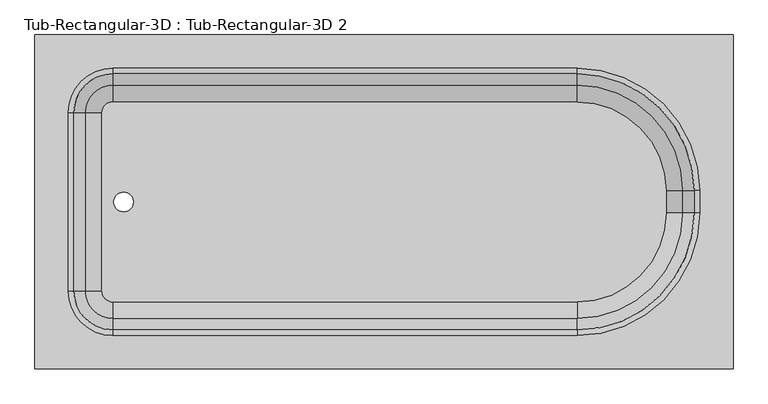
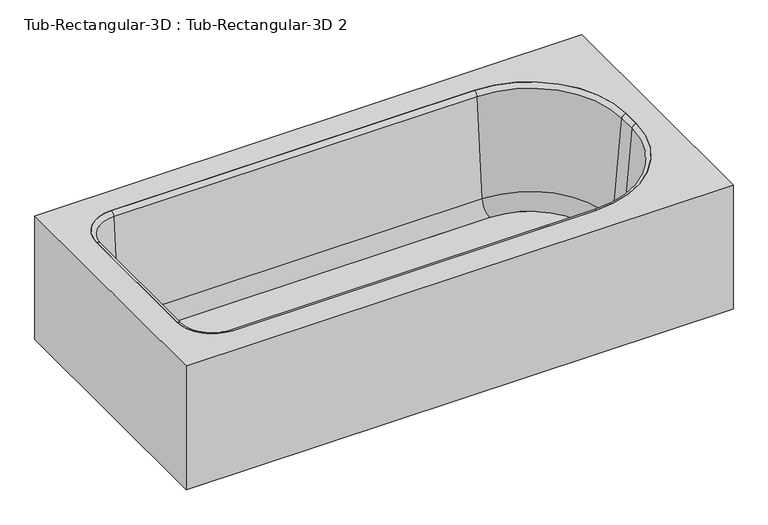
"""IFC4 building model written with IfcOpenShell, lengths in millimetres: flow terminal geometry, Tub-Rectangular-3D : Tub-Rectangular-3D 2."""

import ifcopenshell
import ifcopenshell.guid

model = None  # the IFC model being written
_history = None  # IfcOwnerHistory: only IFC2X3 demands one
_inside = {}  # id of a spatial element -> (the spatial element, [elements in it])
_under = {}  # id of a project, library or spatial element -> (it, [spatial elements below it])
_declared = {}  # id of a project -> (the project, [libraries it declares])
_typed = {}  # id of a type object -> (the type object, [elements of that type])
_made_of = {}  # id of a material, layer set ... -> (it, [elements and type objects made of it])


def new_model(schema):
    """Start an empty IFC model of exactly this schema.

    Asked for "IFC4X3", IfcOpenShell would pick the latest addendum, in which some entities
    have other attributes; the version numbers below select the first issue.
    IFC2X3 requires an IfcOwnerHistory on every rooted entity: one is made here for all.
    """
    global model, _history
    if schema == "IFC4X3":
        model = ifcopenshell.file(schema_version=(4, 3, 0, 0))
    else:
        model = ifcopenshell.file(schema=schema)
    _inside.clear()
    _under.clear()
    _declared.clear()
    _typed.clear()
    _made_of.clear()
    _history = None
    if model.schema == "IFC2X3":
        org = make("IfcOrganization", Name="unknown")
        user = make(
            "IfcPersonAndOrganization",
            ThePerson=make("IfcPerson", FamilyName="unknown"),
            TheOrganization=org,
        )
        app = make(
            "IfcApplication",
            ApplicationDeveloper=org,
            Version="unknown",
            ApplicationFullName="unknown",
            ApplicationIdentifier="unknown",
        )
        _history = make(
            "IfcOwnerHistory",
            OwningUser=user,
            OwningApplication=app,
            ChangeAction="ADDED",
            CreationDate=0,
        )
    return model


def make(cls, **values):
    """One entity of the class cls with the attributes given. An attribute that is None is left unset."""
    return model.create_entity(
        cls, **{name: value for name, value in values.items() if value is not None}
    )


def rooted(cls, **values):
    """An entity with a GlobalId (a new one), such as an element, a storey or a relation."""
    return make(cls, GlobalId=ifcopenshell.guid.new(), OwnerHistory=_history, **values)


def si_unit(unit_type, name, prefix=None):
    """IfcSIUnit, for example si_unit("LENGTHUNIT", "METRE", prefix="MILLI")."""
    return make("IfcSIUnit", UnitType=unit_type, Prefix=prefix, Name=name)


def assignment(units):
    """IfcUnitAssignment: the units of a project."""
    return None if units is None else make("IfcUnitAssignment", Units=units)


def point(xyz):
    """IfcCartesianPoint."""
    return None if xyz is None else make("IfcCartesianPoint", Coordinates=xyz)


def direction(xyz):
    """IfcDirection."""
    return None if xyz is None else make("IfcDirection", DirectionRatios=xyz)


def frame(location, z_axis=None, x_axis=None):
    """IfcAxis2Placement3D, a coordinate frame: its origin and axes. An axis left out is left unset."""
    return make(
        "IfcAxis2Placement3D",
        Location=point(location),
        Axis=direction(z_axis),
        RefDirection=direction(x_axis),
    )


def frame_2d(location, x_axis=None):
    """IfcAxis2Placement2D, a coordinate frame in the plane: its origin and x axis."""
    return make(
        "IfcAxis2Placement2D", Location=point(location), RefDirection=direction(x_axis)
    )


def origin():
    """The frame at (0, 0, 0) with its axes left unset."""
    return frame((0.0, 0.0, 0.0))


def place(relative_to, where):
    """IfcLocalPlacement: puts the frame where relative to a parent placement (None: the world)."""
    return make(
        "IfcLocalPlacement", PlacementRelTo=relative_to, RelativePlacement=where
    )


def context(
    kind, dimensions, precision=None, world=None, true_north=None, identifier=None
):
    """IfcGeometricRepresentationContext, for example the 3D "Model" context."""
    return make(
        "IfcGeometricRepresentationContext",
        ContextIdentifier=identifier,
        ContextType=kind,
        CoordinateSpaceDimension=dimensions,
        Precision=precision,
        WorldCoordinateSystem=world,
        TrueNorth=true_north,
    )


def project(units=None, contexts=None):
    """IfcProject with its units and contexts."""
    return rooted(
        "IfcProject",
        Name="project",
        RepresentationContexts=contexts,
        UnitsInContext=assignment(units),
    )


def spatial(cls, under=None, at=None, **own):
    """A site, building, storey or space (cls), placed at a placement, below another one or the project."""
    s = rooted(cls, ObjectPlacement=at, **own)
    if under is not None:
        _under.setdefault(under.id(), (under, []))[1].append(s)
    return s


def polyline(points):
    """IfcPolyline through the points."""
    return make("IfcPolyline", Points=[point(p) for p in points])


def circle_curve(where, radius):
    """IfcCircle in the frame where."""
    return make("IfcCircle", Position=where, Radius=radius)


def ellipse_curve(where, semi_axis1, semi_axis2):
    """IfcEllipse in the frame where."""
    return make(
        "IfcEllipse", Position=where, SemiAxis1=semi_axis1, SemiAxis2=semi_axis2
    )


def trimmed(basis, trim1, trim2, sense, master):
    """IfcTrimmedCurve: the piece of a basis curve between two trims."""
    return make(
        "IfcTrimmedCurve",
        BasisCurve=basis,
        Trim1=trim1,
        Trim2=trim2,
        SenseAgreement=sense,
        MasterRepresentation=master,
    )


def segment(curve, same_sense, transition):
    """IfcCompositeCurveSegment."""
    return make(
        "IfcCompositeCurveSegment",
        Transition=transition,
        SameSense=same_sense,
        ParentCurve=curve,
    )


def composite_curve(segments, self_intersect=None):
    """IfcCompositeCurve: segments joined end to end."""
    return make("IfcCompositeCurve", Segments=segments, SelfIntersect=self_intersect)


def outline(outer, holes=None, kind="AREA"):
    """IfcArbitraryClosedProfileDef: a profile drawn as a closed curve; with holes, ...WithVoids."""
    if holes is None:
        return make("IfcArbitraryClosedProfileDef", ProfileType=kind, OuterCurve=outer)
    return make(
        "IfcArbitraryProfileDefWithVoids",
        ProfileType=kind,
        OuterCurve=outer,
        InnerCurves=holes,
    )


def extrude(swept, where, along, depth):
    """IfcExtrudedAreaSolid: the profile swept, set in the frame where, extruded along a direction by depth."""
    return make(
        "IfcExtrudedAreaSolid",
        SweptArea=swept,
        Position=where,
        ExtrudedDirection=direction(along),
        Depth=depth,
    )


def shape(context_of_items, identifier, shape_type, items):
    """IfcShapeRepresentation: the items that make up one representation, for example the "Body"."""
    return make(
        "IfcShapeRepresentation",
        ContextOfItems=context_of_items,
        RepresentationIdentifier=identifier,
        RepresentationType=shape_type,
        Items=items,
    )


def source(mapping_origin, context_of_items, identifier, shape_type, items):
    """IfcRepresentationMap: a shape defined once, which mapped items show again and again."""
    return make(
        "IfcRepresentationMap",
        MappingOrigin=mapping_origin,
        MappedRepresentation=shape(context_of_items, identifier, shape_type, items),
    )


def transform(
    local_origin,
    x_axis=None,
    y_axis=None,
    z_axis=None,
    scale=None,
    scale2=None,
    scale3=None,
    uniform=True,
):
    """IfcCartesianTransformationOperator3D, or its non-uniform kind. x_axis, y_axis, z_axis: its Axis1, 2, 3."""
    if uniform:
        return make(
            "IfcCartesianTransformationOperator3D",
            Axis1=direction(x_axis),
            Axis2=direction(y_axis),
            LocalOrigin=point(local_origin),
            Scale=scale,
            Axis3=direction(z_axis),
        )
    return make(
        "IfcCartesianTransformationOperator3DnonUniform",
        Axis1=direction(x_axis),
        Axis2=direction(y_axis),
        LocalOrigin=point(local_origin),
        Scale=scale,
        Axis3=direction(z_axis),
        Scale2=scale2,
        Scale3=scale3,
    )


def mapped(mapping_source, mapping_target):
    """IfcMappedItem: shows the shape of a source again, moved by a transform."""
    return make(
        "IfcMappedItem", MappingSource=mapping_source, MappingTarget=mapping_target
    )


def made_of(thing, what):
    """Note that an element or type object is made of a material, layer set ...; save() writes the relation."""
    if what is not None:
        _made_of.setdefault(what.id(), (what, []))[1].append(thing)
    return thing


def element(
    cls,
    number,
    at=None,
    inside=None,
    cuts=None,
    type_object=None,
    material=None,
    context=None,
    identifier="Body",
    shape_type=None,
    held_by="IfcProductDefinitionShape",
    body=None,
    shapes=None,
    **own,
):
    """One element of the class cls, such as IfcWall. Its Tag is "e" and its number.

    at: its placement. inside: the storey or other place that contains it. cuts: it is an
    opening in that element (IfcRelVoidsElement). A single representation is given by context,
    identifier, shape_type and body (its items); several are given by shapes. held_by: the class
    of the entity that holds the representations. save() writes the other relations.
    """
    e = rooted(cls, Tag="e%d" % number, ObjectPlacement=at, **own)
    if body is not None:
        shapes = [shape(context, identifier, shape_type, body)]
    if shapes is not None:
        e.Representation = make(held_by, Representations=shapes)
    if inside is not None:
        _inside.setdefault(inside.id(), (inside, []))[1].append(e)
    if cuts is not None:
        rooted(
            "IfcRelVoidsElement", RelatingBuildingElement=cuts, RelatedOpeningElement=e
        )
    if type_object is not None:
        _typed.setdefault(type_object.id(), (type_object, []))[1].append(e)
    return made_of(e, material)


def aggregate(whole, parts):
    """IfcRelAggregates: a whole, such as a stair, and the parts it consists of."""
    return rooted("IfcRelAggregates", RelatingObject=whole, RelatedObjects=parts)


def save(model, path):
    """Write the relations noted so far, then the file.

    IfcRelAggregates (storeys below a building ...), IfcRelContainedInSpatialStructure (elements
    in a storey), IfcRelDefinesByType, IfcRelAssociatesMaterial and IfcRelDeclares: one each for
    every whole, place, type object, material and project.
    """
    for whole, parts in _under.values():
        aggregate(whole, parts)
    for where, things in _inside.values():
        rooted(
            "IfcRelContainedInSpatialStructure",
            RelatedElements=things,
            RelatingStructure=where,
        )
    for kind, things in _typed.values():
        rooted("IfcRelDefinesByType", RelatedObjects=things, RelatingType=kind)
    for what, things in _made_of.values():
        rooted("IfcRelAssociatesMaterial", RelatedObjects=things, RelatingMaterial=what)
    for by, libraries in _declared.values():
        rooted("IfcRelDeclares", RelatingContext=by, RelatedDefinitions=libraries)
    model.write(path)


def plane_surface(at):
    """IfcPlane: the flat surface through the origin of the frame at, square to its z axis."""
    return make("IfcPlane", Position=at)


def cylinder_surface(at, radius):
    """IfcCylindricalSurface: all points at the distance radius from the z axis of the frame at."""
    return make("IfcCylindricalSurface", Position=at, Radius=radius)


def revolved_surface(curve, axis_point, axis_direction):
    """IfcSurfaceOfRevolution: the curve turned about the line through axis_point along axis_direction."""
    return make(
        "IfcSurfaceOfRevolution",
        SweptCurve=make("IfcArbitraryOpenProfileDef", ProfileType="CURVE", Curve=curve),
        AxisPosition=make("IfcAxis1Placement", Location=point(axis_point), Axis=direction(axis_direction)),
    )


def advanced_brep(points, edges, surfaces, faces):
    """IfcAdvancedBrep: a solid bounded by faces that lie on surfaces and meet in shared edges.

    An edge is (start, end): straight between two places in points (the first is 0);
    or (start, end, curve); or (start, end, curve, False) where it runs against its curve.
    A face is (place in surfaces, loops), or (place, loops, False) where it looks against
    its surface's normal. A loop lists edges by number (the first is 1), with a minus sign
    where the edge is run from its end to its start. The first loop is the outer one.
    """
    corners = [point(p) for p in points]
    vertices = [make("IfcVertexPoint", VertexGeometry=c) for c in corners]
    made = []
    for start, end, *more in edges:
        made.append(
            make(
                "IfcEdgeCurve",
                EdgeStart=vertices[start],
                EdgeEnd=vertices[end],
                EdgeGeometry=more[0] if more else make("IfcPolyline", Points=[corners[start], corners[end]]),
                SameSense=more[1] if len(more) > 1 else True,
            )
        )
    hull = []
    for where, loops, *sense in faces:
        bounds = []
        for j, loop in enumerate(loops):
            ring = [make("IfcOrientedEdge", EdgeElement=made[abs(k) - 1], Orientation=k > 0) for k in loop]
            bounds.append(
                make(
                    "IfcFaceOuterBound" if j == 0 else "IfcFaceBound",
                    Bound=make("IfcEdgeLoop", EdgeList=ring),
                    Orientation=True,
                )
            )
        hull.append(make("IfcAdvancedFace", Bounds=bounds, FaceSurface=surfaces[where], SameSense=sense[0] if sense else True))
    return make("IfcAdvancedBrep", Outer=make("IfcClosedShell", CfsFaces=hull))


def tub_rectangular_3d_tub_rectangular_3d_2_b18e5bc2(model_context):
    return source(origin(), model_context, "Body", "SolidModel", [
        advanced_brep(
        [(480.0720313, 830.2625, 381.0), (-1110.6029687, 830.2625, 381.0), (-1110.6029687, 68.2625, 381.0), (480.0720313, 68.2625, 381.0), (-932.8029687, 754.0625, 381.0), (124.4720313, 754.0625, 381.0), (403.8720313, 474.6625, 381.0), (403.8720313, 423.8625, 381.0), (124.4720313, 144.4625, 381.0), (-932.8029687, 144.4625, 381.0), (-1034.4029687, 246.0625, 381.0), (-1034.4029687, 652.4625, 381.0), (461.0220313, 811.2125, 361.95), (461.0220313, 87.3125, 361.95), (-1091.5529687, 87.3125, 361.95), (-1091.5529687, 811.2125, 361.95), (-932.8029687, 754.0625, 361.95), (-1034.4029687, 652.4625, 361.95), (-1034.4029687, 246.0625, 361.95), (-932.8029687, 144.4625, 361.95), (124.4720313, 144.4625, 361.95), (403.8720313, 423.8625, 361.95), (403.8720313, 474.6625, 361.95), (124.4720313, 754.0625, 361.95), (480.0720313, 830.2625, 0.0), (-1110.6029687, 830.2625, 0.0), (-1110.6029687, 68.2625, 0.0), (480.0720313, 68.2625, 0.0), (461.0220313, 811.2125, 0.0), (-1091.5529687, 811.2125, 0.0), (-1091.5529687, 87.3125, 0.0), (461.0220313, 87.3125, 0.0)],
        [
            (0, 1),
            (1, 2),
            (2, 3),
            (3, 0),
            (4, 5),
            (5, 6, circle_curve(frame((124.4720313, 474.6625, 381.0), z_axis=(0.0, 0.0, -1.0), x_axis=(0.0, 1.0, 0.0)), 279.4)),
            (6, 7),
            (7, 8, circle_curve(frame((124.4720313, 423.8625, 381.0), z_axis=(0.0, 0.0, -1.0), x_axis=(0.0, 1.0, 0.0)), 279.4)),
            (8, 9),
            (9, 10, circle_curve(frame((-932.8029687, 246.0625, 381.0), z_axis=(0.0, 0.0, -1.0), x_axis=(0.0, 1.0, 0.0)), 101.6)),
            (10, 11),
            (11, 4, circle_curve(frame((-932.8029687, 652.4625, 381.0), z_axis=(0.0, 0.0, -1.0), x_axis=(0.0, 1.0, 0.0)), 101.6)),
            (12, 13),
            (13, 14),
            (14, 15),
            (15, 12),
            (16, 17, circle_curve(frame((-932.8029687, 652.4625, 361.95), z_axis=(0.0, 0.0, 1.0), x_axis=(0.0, 1.0, 0.0)), 101.6)),
            (17, 18),
            (18, 19, circle_curve(frame((-932.8029687, 246.0625, 361.95), z_axis=(0.0, 0.0, 1.0), x_axis=(0.0, 1.0, 0.0)), 101.6)),
            (19, 20),
            (20, 21, circle_curve(frame((124.4720313, 423.8625, 361.95), z_axis=(0.0, 0.0, 1.0), x_axis=(0.0, 1.0, 0.0)), 279.4)),
            (21, 22),
            (22, 23, circle_curve(frame((124.4720313, 474.6625, 361.95), z_axis=(0.0, 0.0, 1.0), x_axis=(0.0, 1.0, 0.0)), 279.4)),
            (23, 16),
            (0, 24),
            (24, 25),
            (25, 1),
            (25, 26),
            (26, 2),
            (26, 27),
            (27, 3),
            (27, 24),
            (4, 16),
            (23, 5),
            (22, 6),
            (21, 7),
            (20, 8),
            (19, 9),
            (18, 10),
            (17, 11),
            (28, 29),
            (29, 30),
            (30, 31),
            (31, 28),
            (31, 13),
            (12, 28),
            (30, 14),
            (29, 15),
        ],
        [
            plane_surface(frame((-1110.6029687, 830.2625, 381.0), z_axis=(0.0, 0.0, 1.0), x_axis=(-1.0, 0.0, 0.0))),
            plane_surface(frame((-1110.6029687, 830.2625, 361.95), z_axis=(0.0, 0.0, -1.0), x_axis=(1.0, 0.0, 0.0))),
            plane_surface(frame((480.0720313, 830.2625, 381.0), z_axis=(0.0, 1.0, 0.0), x_axis=(0.0, 0.0, -1.0))),
            plane_surface(frame((-1110.6029687, 830.2625, 381.0), z_axis=(-1.0, 0.0, 0.0), x_axis=(0.0, 0.0, -1.0))),
            plane_surface(frame((-1110.6029687, 68.2625, 381.0), z_axis=(0.0, -1.0, 0.0), x_axis=(0.0, 0.0, -1.0))),
            plane_surface(frame((480.0720313, 68.2625, 381.0), z_axis=(1.0, 0.0, 0.0), x_axis=(0.0, 0.0, -1.0))),
            plane_surface(frame((-932.8029687, 754.0625, 381.0), z_axis=(0.0, -1.0, 0.0), x_axis=(0.0, 0.0, -1.0))),
            revolved_surface(polyline([(124.4720313, 754.0625, 361.95), (124.4720313, 754.0625, 381.0)]), (124.4720313, 474.6625, 381.0), (0.0, 0.0, -1.0)),
            plane_surface(frame((403.8720313, 474.6625, 381.0), z_axis=(-1.0, 0.0, 0.0), x_axis=(0.0, 0.0, -1.0))),
            revolved_surface(polyline([(124.4720313, 703.2625, 361.95), (124.4720313, 703.2625, 381.0)]), (124.4720313, 423.8625, 381.0), (0.0, 0.0, -1.0)),
            plane_surface(frame((124.4720313, 144.4625, 381.0), z_axis=(0.0, 1.0, 0.0), x_axis=(0.0, 0.0, -1.0))),
            revolved_surface(polyline([(-932.8029687, 347.6625, 361.95), (-932.8029687, 347.6625, 381.0)]), (-932.8029687, 246.0625, 381.0), (0.0, 0.0, -1.0)),
            plane_surface(frame((-1034.4029687, 246.0625, 381.0), z_axis=(1.0, 0.0, 0.0), x_axis=(0.0, 0.0, -1.0))),
            revolved_surface(polyline([(-932.8029687, 754.0625, 361.95), (-932.8029687, 754.0625, 381.0)]), (-932.8029687, 652.4625, 381.0), (0.0, 0.0, -1.0)),
            plane_surface(frame((-1110.6029687, 830.2625, 0.0), z_axis=(0.0, 0.0, -1.0), x_axis=(1.0, 0.0, 0.0))),
            plane_surface(frame((461.0220313, 811.2125, 361.95), z_axis=(-1.0, 0.0, 0.0), x_axis=(0.0, 0.0, -1.0))),
            plane_surface(frame((461.0220313, 87.3125, 361.95), z_axis=(0.0, 1.0, 0.0), x_axis=(0.0, 0.0, -1.0))),
            plane_surface(frame((-1091.5529687, 87.3125, 361.95), z_axis=(1.0, 0.0, 0.0), x_axis=(0.0, 0.0, -1.0))),
            plane_surface(frame((-1091.5529687, 811.2125, 361.95), z_axis=(0.0, -1.0, 0.0), x_axis=(0.0, 0.0, -1.0))),
        ],
        [
            (0, [[1, 2, 3, 4], [5, 6, 7, 8, 9, 10, 11, 12]]),
            (1, [[13, 14, 15, 16], [17, 18, 19, 20, 21, 22, 23, 24]]),
            (2, [[-1, 25, 26, 27]]),
            (3, [[-2, -27, 28, 29]]),
            (4, [[-3, -29, 30, 31]]),
            (5, [[-25, -4, -31, 32]]),
            (6, [[-5, 33, -24, 34]]),
            (7, [[-6, -34, -23, 35]]),
            (8, [[-7, -35, -22, 36]]),
            (9, [[-8, -36, -21, 37]]),
            (10, [[-9, -37, -20, 38]]),
            (11, [[-10, -38, -19, 39]]),
            (12, [[-11, -39, -18, 40]]),
            (13, [[-12, -40, -17, -33]]),
            (14, [[-32, -30, -28, -26], [41, 42, 43, 44]]),
            (15, [[-44, 45, -13, 46]]),
            (16, [[-43, 47, -14, -45]]),
            (17, [[-42, 48, -15, -47]]),
            (18, [[-41, -46, -16, -48]]),
        ],
    ),
        extrude(outline(composite_curve([segment(trimmed(circle_curve(frame_2d((124.4720313, 474.6625)), 202.7964741), [point((124.4720313, 677.4589741))], [point((327.2685054, 474.6625))], False, "CARTESIAN"), True, "CONTINUOUS"), segment(polyline([(327.2685054, 474.6625), (327.2685054, 423.8625)]), True, "CONTINUOUS"), segment(trimmed(circle_curve(frame_2d((124.4720313, 423.8625)), 202.7964741), [point((327.2685054, 423.8625))], [point((124.4720313, 221.0660259))], False, "CARTESIAN"), True, "CONTINUOUS"), segment(polyline([(124.4720313, 221.0660259), (-932.8029687, 221.0660259)]), True, "CONTINUOUS"), segment(trimmed(circle_curve(frame_2d((-932.8029687, 246.0625)), 24.9964741), [point((-932.8029687, 221.0660259))], [point((-957.7994428, 246.0625))], False, "CARTESIAN"), True, "CONTINUOUS"), segment(polyline([(-957.7994428, 246.0625), (-957.7994428, 652.4625)]), True, "CONTINUOUS"), segment(trimmed(circle_curve(frame_2d((-932.8029687, 652.4625)), 24.9964741), [point((-957.7994428, 652.4625))], [point((-932.8029687, 677.4589741))], False, "CARTESIAN"), True, "CONTINUOUS"), segment(polyline([(-932.8029687, 677.4589741), (124.4720313, 677.4589741)]), True, "CONTINUOUS")], self_intersect=False), holes=[composite_curve([segment(trimmed(circle_curve(frame_2d((-908.510206, 449.2625)), 22.225), [point((-908.510206, 471.4875))], [point((-908.510206, 427.0375))], True, "CARTESIAN"), True, "CONTINUOUS"), segment(trimmed(circle_curve(frame_2d((-908.510206, 449.2625)), 22.225), [point((-908.510206, 427.0375))], [point((-908.510206, 471.4875))], True, "CARTESIAN"), True, "CONTINUOUS")], self_intersect=False)]), frame((0.0, 0.0, 16.863573), z_axis=(0.0, 0.0, 1.0), x_axis=(1.0, 0.0, 0.0)), (0.0, 0.0, 1.0), 19.05),
        advanced_brep(
        [(-995.7544608, 652.4625, 70.6929392), (-932.8029687, 715.4139921, 70.6929392), (-932.8029687, 741.5845035, 369.8232535), (-1021.9249722, 652.4625, 369.8232535), (-957.7994428, 652.4625, 35.913573), (-932.8029687, 677.4589741, 35.913573), (-957.7994428, 652.4625, 16.863573), (-932.8029687, 677.4589741, 16.863573), (-1034.4029687, 652.4625, 16.863573), (-932.8029687, 754.0625, 16.863573), (-1034.4029687, 652.4625, 381.0), (-932.8029687, 754.0625, 381.0), (-1021.9249722, 246.0625, 369.8232535), (-995.7544608, 246.0625, 70.6929392), (-957.7994428, 246.0625, 35.913573), (-957.7994428, 246.0625, 16.863573), (-1034.4029687, 246.0625, 16.863573), (-1034.4029687, 246.0625, 381.0), (-932.8029687, 183.1110079, 70.6929392), (-932.8029687, 156.9404965, 369.8232535), (-932.8029687, 221.0660259, 35.913573), (-932.8029687, 221.0660259, 16.863573), (-932.8029687, 144.4625, 16.863573), (-932.8029687, 144.4625, 381.0), (124.4720313, 156.9404965, 369.8232535), (124.4720313, 183.1110079, 70.6929392), (124.4720313, 221.0660259, 35.913573), (124.4720313, 221.0660259, 16.863573), (124.4720313, 144.4625, 16.863573), (124.4720313, 144.4625, 381.0), (365.2235234, 423.8625, 70.6929392), (391.3940348, 423.8625, 369.8232535), (327.2685054, 423.8625, 35.913573), (327.2685054, 423.8625, 16.863573), (403.8720313, 423.8625, 16.863573), (403.8720313, 423.8625, 381.0), (391.3940348, 474.6625, 369.8232535), (365.2235234, 474.6625, 70.6929392), (327.2685054, 474.6625, 35.913573), (327.2685054, 474.6625, 16.863573), (403.8720313, 474.6625, 16.863573), (403.8720313, 474.6625, 381.0), (124.4720313, 715.4139921, 70.6929392), (124.4720313, 741.5845035, 369.8232535), (124.4720313, 677.4589741, 35.913573), (124.4720313, 677.4589741, 16.863573), (124.4720313, 754.0625, 16.863573), (124.4720313, 754.0625, 381.0)],
        [
            (0, 1, circle_curve(frame((-932.8029687, 652.4625, 70.6929392), z_axis=(0.0, 0.0, -1.0), x_axis=(0.0, 1.0, 0.0)), 62.9514921)),
            (1, 2),
            (2, 3, circle_curve(frame((-932.8029687, 652.4625, 369.8232535), z_axis=(0.0, 0.0, 1.0), x_axis=(0.0, 1.0, 0.0)), 89.1220035)),
            (3, 0),
            (4, 5, circle_curve(frame((-932.8029687, 652.4625, 35.913573), z_axis=(0.0, 0.0, -1.0), x_axis=(0.0, 1.0, 0.0)), 24.9964741)),
            (5, 1, circle_curve(frame((-932.8029687, 677.4589741, 74.013573), z_axis=(1.0, 0.0, 0.0), x_axis=(0.0, -1.0, 0.0)), 38.1)),
            (0, 4, circle_curve(frame((-957.7994428, 652.4625, 74.013573), z_axis=(0.0, -1.0, 0.0), x_axis=(1.0, 0.0, 0.0)), 38.1)),
            (6, 7, circle_curve(frame((-932.8029687, 652.4625, 16.863573), z_axis=(0.0, 0.0, -1.0), x_axis=(0.0, 1.0, 0.0)), 24.9964741)),
            (7, 5),
            (4, 6),
            (8, 9, circle_curve(frame((-932.8029687, 652.4625, 16.863573), z_axis=(0.0, 0.0, -1.0), x_axis=(0.0, 1.0, 0.0)), 101.6)),
            (9, 7),
            (6, 8),
            (10, 11, circle_curve(frame((-932.8029687, 652.4625, 381.0), z_axis=(0.0, 0.0, -1.0), x_axis=(0.0, 1.0, 0.0)), 101.6)),
            (11, 9),
            (8, 10),
            (2, 11, circle_curve(frame((-932.8029687, 754.0625, 368.4462547), z_axis=(-1.0, 0.0, 0.0), x_axis=(0.0, -1.0, 0.0)), 12.5537453)),
            (10, 3, circle_curve(frame((-1034.4029687, 652.4625, 368.4462547), z_axis=(0.0, 1.0, 0.0), x_axis=(1.0, 0.0, 0.0)), 12.5537453)),
            (3, 12),
            (12, 13),
            (13, 0),
            (13, 14, circle_curve(frame((-957.7994428, 246.0625, 74.013573), z_axis=(0.0, -1.0, 0.0), x_axis=(1.0, 0.0, 0.0)), 38.1)),
            (14, 4),
            (14, 15),
            (15, 6),
            (15, 16),
            (16, 8),
            (16, 17),
            (17, 10),
            (17, 12, circle_curve(frame((-1034.4029687, 246.0625, 368.4462547), z_axis=(0.0, 1.0, 0.0), x_axis=(1.0, 0.0, 0.0)), 12.5537453)),
            (18, 13, circle_curve(frame((-932.8029687, 246.0625, 70.6929392), z_axis=(0.0, 0.0, -1.0), x_axis=(-1.0, 0.0, 0.0)), 62.9514921)),
            (12, 19, circle_curve(frame((-932.8029687, 246.0625, 369.8232535), z_axis=(0.0, 0.0, 1.0), x_axis=(-1.0, 0.0, 0.0)), 89.1220035)),
            (19, 18),
            (20, 14, circle_curve(frame((-932.8029687, 246.0625, 35.913573), z_axis=(0.0, 0.0, -1.0), x_axis=(-1.0, 0.0, 0.0)), 24.9964741)),
            (18, 20, circle_curve(frame((-932.8029687, 221.0660259, 74.013573), z_axis=(1.0, 0.0, 0.0), x_axis=(0.0, 1.0, 0.0)), 38.1)),
            (21, 15, circle_curve(frame((-932.8029687, 246.0625, 16.863573), z_axis=(0.0, 0.0, -1.0), x_axis=(-1.0, 0.0, 0.0)), 24.9964741)),
            (20, 21),
            (22, 16, circle_curve(frame((-932.8029687, 246.0625, 16.863573), z_axis=(0.0, 0.0, -1.0), x_axis=(-1.0, 0.0, 0.0)), 101.6)),
            (21, 22),
            (23, 17, circle_curve(frame((-932.8029687, 246.0625, 381.0), z_axis=(0.0, 0.0, -1.0), x_axis=(-1.0, 0.0, 0.0)), 101.6)),
            (22, 23),
            (23, 19, circle_curve(frame((-932.8029687, 144.4625, 368.4462547), z_axis=(-1.0, 0.0, 0.0), x_axis=(0.0, 1.0, 0.0)), 12.5537453)),
            (19, 24),
            (24, 25),
            (25, 18),
            (25, 26, circle_curve(frame((124.4720313, 221.0660259, 74.013573), z_axis=(1.0, 0.0, 0.0), x_axis=(0.0, 1.0, 0.0)), 38.1)),
            (26, 20),
            (26, 27),
            (27, 21),
            (27, 28),
            (28, 22),
            (28, 29),
            (29, 23),
            (29, 24, circle_curve(frame((124.4720313, 144.4625, 368.4462547), z_axis=(-1.0, 0.0, 0.0), x_axis=(0.0, 1.0, 0.0)), 12.5537453)),
            (30, 25, circle_curve(frame((124.4720313, 423.8625, 70.6929392), z_axis=(0.0, 0.0, -1.0), x_axis=(0.0, -1.0, 0.0)), 240.7514921)),
            (24, 31, circle_curve(frame((124.4720313, 423.8625, 369.8232535), z_axis=(0.0, 0.0, 1.0), x_axis=(0.0, -1.0, 0.0)), 266.9220035)),
            (31, 30),
            (32, 26, circle_curve(frame((124.4720313, 423.8625, 35.913573), z_axis=(0.0, 0.0, -1.0), x_axis=(0.0, -1.0, 0.0)), 202.7964741)),
            (30, 32, circle_curve(frame((327.2685054, 423.8625, 74.013573), z_axis=(0.0, 1.0, 0.0), x_axis=(-1.0, 0.0, 0.0)), 38.1)),
            (33, 27, circle_curve(frame((124.4720313, 423.8625, 16.863573), z_axis=(0.0, 0.0, -1.0), x_axis=(0.0, -1.0, 0.0)), 202.7964741)),
            (32, 33),
            (34, 28, circle_curve(frame((124.4720313, 423.8625, 16.863573), z_axis=(0.0, 0.0, -1.0), x_axis=(0.0, -1.0, 0.0)), 279.4)),
            (33, 34),
            (35, 29, circle_curve(frame((124.4720313, 423.8625, 381.0), z_axis=(0.0, 0.0, -1.0), x_axis=(0.0, -1.0, 0.0)), 279.4)),
            (34, 35),
            (35, 31, circle_curve(frame((403.8720313, 423.8625, 368.4462547), z_axis=(0.0, -1.0, 0.0), x_axis=(-1.0, 0.0, 0.0)), 12.5537453)),
            (31, 36),
            (36, 37),
            (37, 30),
            (37, 38, circle_curve(frame((327.2685054, 474.6625, 74.013573), z_axis=(0.0, 1.0, 0.0), x_axis=(-1.0, 0.0, 0.0)), 38.1)),
            (38, 32),
            (38, 39),
            (39, 33),
            (39, 40),
            (40, 34),
            (40, 41),
            (41, 35),
            (41, 36, circle_curve(frame((403.8720313, 474.6625, 368.4462547), z_axis=(0.0, -1.0, 0.0), x_axis=(-1.0, 0.0, 0.0)), 12.5537453)),
            (42, 37, circle_curve(frame((124.4720313, 474.6625, 70.6929392), z_axis=(0.0, 0.0, -1.0), x_axis=(1.0, 0.0, 0.0)), 240.7514921)),
            (36, 43, circle_curve(frame((124.4720313, 474.6625, 369.8232535), z_axis=(0.0, 0.0, 1.0), x_axis=(1.0, 0.0, 0.0)), 266.9220035)),
            (43, 42),
            (44, 38, circle_curve(frame((124.4720313, 474.6625, 35.913573), z_axis=(0.0, 0.0, -1.0), x_axis=(1.0, 0.0, 0.0)), 202.7964741)),
            (42, 44, circle_curve(frame((124.4720313, 677.4589741, 74.013573), z_axis=(-1.0, 0.0, 0.0), x_axis=(0.0, -1.0, 0.0)), 38.1)),
            (45, 39, circle_curve(frame((124.4720313, 474.6625, 16.863573), z_axis=(0.0, 0.0, -1.0), x_axis=(1.0, 0.0, 0.0)), 202.7964741)),
            (44, 45),
            (46, 40, circle_curve(frame((124.4720313, 474.6625, 16.863573), z_axis=(0.0, 0.0, -1.0), x_axis=(1.0, 0.0, 0.0)), 279.4)),
            (45, 46),
            (47, 41, circle_curve(frame((124.4720313, 474.6625, 381.0), z_axis=(0.0, 0.0, -1.0), x_axis=(1.0, 0.0, 0.0)), 279.4)),
            (46, 47),
            (47, 43, circle_curve(frame((124.4720313, 754.0625, 368.4462547), z_axis=(1.0, 0.0, 0.0), x_axis=(0.0, -1.0, 0.0)), 12.5537453)),
            (43, 2),
            (1, 42),
            (5, 44),
            (7, 45),
            (9, 46),
            (11, 47),
        ],
        [
            revolved_surface(polyline([(-932.8029687, 741.5845035, 369.8232535), (-932.8029687, 715.4139921, 70.6929392)]), (-932.8029687, 652.4625, 381.0), (0.0, 0.0, 1.0)),
            revolved_surface(trimmed(ellipse_curve(frame((-932.8029687, 677.4589741, 74.013573), z_axis=(-1.0, 0.0, 0.0), x_axis=(0.0, -1.0, 0.0)), 38.1, 38.1), [point((-932.8029687, 715.4139921, 70.6929392))], [point((-932.8029687, 677.4589741, 35.913573))], True, "CARTESIAN"), (-932.8029687, 652.4625, 381.0), (0.0, 0.0, 1.0)),
            revolved_surface(polyline([(-932.8029687, 677.4589741, 35.913572999999985), (-932.8029687, 677.4589741, 16.863572999999974)]), (-932.8029687, 652.4625, 381.0), (0.0, 0.0, 1.0)),
            plane_surface(frame((-932.8029687, 652.4625, 16.863573), z_axis=(0.0, 0.0, -1.0), x_axis=(0.0, 1.0, 0.0))),
            cylinder_surface(frame((-932.8029687, 652.4625, 381.0), z_axis=(0.0, 0.0, 1.0), x_axis=(0.0, 1.0, 0.0)), 101.6),
            revolved_surface(trimmed(ellipse_curve(frame((-932.8029687, 754.0625, 368.4462547), z_axis=(1.0, 0.0, 0.0), x_axis=(0.0, -1.0, 0.0)), 12.5537453, 12.5537453), [point((-932.8029687, 754.0625, 381.0))], [point((-932.8029687, 741.5845035, 369.8232535))], True, "CARTESIAN"), (-932.8029687, 652.4625, 381.0), (0.0, 0.0, 1.0)),
            plane_surface(frame((-1021.9249722, 652.4625, 369.8232535), z_axis=(0.9961946980917458, 0.0, 0.08715574274765595), x_axis=(0.0, -1.0, 0.0))),
            revolved_surface(polyline([(-919.6994427999999, 246.0625, 74.013573), (-919.6994427999999, 652.4625, 74.013573)]), (-957.7994428, 652.4625, 74.013573), (0.0, -1.0, 0.0)),
            plane_surface(frame((-957.7994428, 652.4625, 35.913573), z_axis=(1.0, 0.0, 0.0), x_axis=(0.0, -1.0, 0.0))),
            plane_surface(frame((-957.7994428, 652.4625, 16.863573), z_axis=(0.0, 0.0, -1.0), x_axis=(0.0, -1.0, 0.0))),
            plane_surface(frame((-1034.4029687, 652.4625, 16.863573), z_axis=(-1.0, 0.0, 0.0), x_axis=(0.0, -1.0, 0.0))),
            cylinder_surface(frame((-1034.4029687, 652.4625, 368.4462547), z_axis=(0.0, 1.0, 0.0), x_axis=(1.0, 0.0, 0.0)), 12.5537453),
            revolved_surface(polyline([(-1021.9249722, 246.0625, 369.8232535), (-995.7544608, 246.0625, 70.6929392)]), (-932.8029687, 246.0625, 381.0), (0.0, 0.0, 1.0)),
            revolved_surface(trimmed(ellipse_curve(frame((-957.7994428, 246.0625, 74.013573), z_axis=(0.0, -1.0, 0.0), x_axis=(1.0, 0.0, 0.0)), 38.1, 38.1), [point((-995.7544608, 246.0625, 70.6929392))], [point((-957.7994428, 246.0625, 35.913573))], True, "CARTESIAN"), (-932.8029687, 246.0625, 381.0), (0.0, 0.0, 1.0)),
            revolved_surface(polyline([(-957.7994428, 246.0625, 35.913572999999985), (-957.7994428, 246.0625, 16.863572999999974)]), (-932.8029687, 246.0625, 381.0), (0.0, 0.0, 1.0)),
            plane_surface(frame((-932.8029687, 246.0625, 16.863573), z_axis=(0.0, 0.0, -1.0), x_axis=(-1.0, 0.0, 0.0))),
            cylinder_surface(frame((-932.8029687, 246.0625, 381.0), z_axis=(0.0, 0.0, 1.0), x_axis=(-1.0, 0.0, 0.0)), 101.6),
            revolved_surface(trimmed(ellipse_curve(frame((-1034.4029687, 246.0625, 368.4462547), z_axis=(0.0, 1.0, 0.0), x_axis=(1.0, 0.0, 0.0)), 12.5537453, 12.5537453), [point((-1034.4029687, 246.0625, 381.0))], [point((-1021.9249722, 246.0625, 369.8232535))], True, "CARTESIAN"), (-932.8029687, 246.0625, 381.0), (0.0, 0.0, 1.0)),
            plane_surface(frame((-932.8029687, 156.9404965, 369.8232535), z_axis=(0.0, 0.9961946980917461, 0.08715574274765271), x_axis=(1.0, 0.0, 0.0))),
            revolved_surface(polyline([(124.47203129999991, 259.1660259, 74.013573), (-932.8029687, 259.1660259, 74.013573)]), (-932.8029687, 221.0660259, 74.013573), (1.0, 0.0, 0.0)),
            plane_surface(frame((-932.8029687, 221.0660259, 35.913573), z_axis=(0.0, 1.0, 0.0), x_axis=(1.0, 0.0, 0.0))),
            plane_surface(frame((-932.8029687, 221.0660259, 16.863573), z_axis=(0.0, 0.0, -1.0), x_axis=(1.0, 0.0, 0.0))),
            plane_surface(frame((-932.8029687, 144.4625, 16.863573), z_axis=(0.0, -1.0, 0.0), x_axis=(1.0, 0.0, 0.0))),
            cylinder_surface(frame((-932.8029687, 144.4625, 368.4462547), z_axis=(-1.0, 0.0, 0.0), x_axis=(0.0, 1.0, 0.0)), 12.5537453),
            revolved_surface(polyline([(124.4720313, 156.9404965, 369.8232535), (124.4720313, 183.1110079, 70.6929392)]), (124.4720313, 423.8625, 381.0), (0.0, 0.0, 1.0)),
            revolved_surface(trimmed(ellipse_curve(frame((124.4720313, 221.0660259, 74.013573), z_axis=(1.0, 0.0, 0.0), x_axis=(0.0, 1.0, 0.0)), 38.1, 38.1), [point((124.4720313, 183.1110079, 70.6929392))], [point((124.4720313, 221.0660259, 35.913573))], True, "CARTESIAN"), (124.4720313, 423.8625, 381.0), (0.0, 0.0, 1.0)),
            revolved_surface(polyline([(124.4720313, 221.0660259, 35.913572999999985), (124.4720313, 221.0660259, 16.863572999999974)]), (124.4720313, 423.8625, 381.0), (0.0, 0.0, 1.0)),
            plane_surface(frame((124.4720313, 423.8625, 16.863573), z_axis=(0.0, 0.0, -1.0), x_axis=(0.0, -1.0, 0.0))),
            cylinder_surface(frame((124.4720313, 423.8625, 381.0), z_axis=(0.0, 0.0, 1.0), x_axis=(0.0, -1.0, 0.0)), 279.4),
            revolved_surface(trimmed(ellipse_curve(frame((124.4720313, 144.4625, 368.4462547), z_axis=(-1.0, 0.0, 0.0), x_axis=(0.0, 1.0, 0.0)), 12.5537453, 12.5537453), [point((124.4720313, 144.4625, 381.0))], [point((124.4720313, 156.9404965, 369.8232535))], True, "CARTESIAN"), (124.4720313, 423.8625, 381.0), (0.0, 0.0, 1.0)),
            plane_surface(frame((391.3940348, 423.8625, 369.8232535), z_axis=(-0.9961946980917464, 0.0, 0.08715574274764948), x_axis=(0.0, 1.0, 0.0))),
            revolved_surface(polyline([(289.16850539999996, 474.6625, 74.013573), (289.16850539999996, 423.8625, 74.013573)]), (327.2685054, 423.8625, 74.013573), (0.0, 1.0, 0.0)),
            plane_surface(frame((327.2685054, 423.8625, 35.913573), z_axis=(-1.0, 0.0, 0.0), x_axis=(0.0, 1.0, 0.0))),
            plane_surface(frame((327.2685054, 423.8625, 16.863573), z_axis=(0.0, 0.0, -1.0), x_axis=(0.0, 1.0, 0.0))),
            plane_surface(frame((403.8720313, 423.8625, 16.863573), z_axis=(1.0, 0.0, 0.0), x_axis=(0.0, 1.0, 0.0))),
            cylinder_surface(frame((403.8720313, 423.8625, 368.4462547), z_axis=(0.0, -1.0, 0.0), x_axis=(-1.0, 0.0, 0.0)), 12.5537453),
            revolved_surface(polyline([(391.3940348, 474.6625, 369.8232535), (365.2235234, 474.6625, 70.6929392)]), (124.4720313, 474.6625, 381.0), (0.0, 0.0, 1.0)),
            revolved_surface(trimmed(ellipse_curve(frame((327.2685054, 474.6625, 74.013573), z_axis=(0.0, 1.0, 0.0), x_axis=(-1.0, 0.0, 0.0)), 38.1, 38.1), [point((365.2235234, 474.6625, 70.6929392))], [point((327.2685054, 474.6625, 35.913573))], True, "CARTESIAN"), (124.4720313, 474.6625, 381.0), (0.0, 0.0, 1.0)),
            revolved_surface(polyline([(327.2685054, 474.6625, 35.913572999999985), (327.2685054, 474.6625, 16.863572999999974)]), (124.4720313, 474.6625, 381.0), (0.0, 0.0, 1.0)),
            plane_surface(frame((124.4720313, 474.6625, 16.863573), z_axis=(0.0, 0.0, -1.0), x_axis=(1.0, 0.0, 0.0))),
            cylinder_surface(frame((124.4720313, 474.6625, 381.0), z_axis=(0.0, 0.0, 1.0), x_axis=(1.0, 0.0, 0.0)), 279.4),
            revolved_surface(trimmed(ellipse_curve(frame((403.8720313, 474.6625, 368.4462547), z_axis=(0.0, -1.0, 0.0), x_axis=(-1.0, 0.0, 0.0)), 12.5537453, 12.5537453), [point((403.8720313, 474.6625, 381.0))], [point((391.3940348, 474.6625, 369.8232535))], True, "CARTESIAN"), (124.4720313, 474.6625, 381.0), (0.0, 0.0, 1.0)),
            plane_surface(frame((124.4720313, 741.5845035, 369.8232535), z_axis=(0.0, -0.9961946980917461, 0.08715574274765271), x_axis=(-1.0, 0.0, 0.0))),
            revolved_surface(polyline([(-932.8029686999998, 639.3589741, 74.013573), (124.4720313, 639.3589741, 74.013573)]), (124.4720313, 677.4589741, 74.013573), (-1.0, 0.0, 0.0)),
            plane_surface(frame((124.4720313, 677.4589741, 35.913573), z_axis=(0.0, -1.0, 0.0), x_axis=(-1.0, 0.0, 0.0))),
            plane_surface(frame((124.4720313, 677.4589741, 16.863573), z_axis=(0.0, 0.0, -1.0), x_axis=(-1.0, 0.0, 0.0))),
            plane_surface(frame((124.4720313, 754.0625, 16.863573), z_axis=(0.0, 1.0, 0.0), x_axis=(-1.0, 0.0, 0.0))),
            cylinder_surface(frame((124.4720313, 754.0625, 368.4462547), z_axis=(1.0, 0.0, 0.0), x_axis=(0.0, -1.0, 0.0)), 12.5537453),
        ],
        [
            (0, [[1, 2, 3, 4]]),
            (1, [[5, 6, -1, 7]]),
            (2, [[8, 9, -5, 10]]),
            (3, [[11, 12, -8, 13]]),
            (4, [[14, 15, -11, 16]]),
            (5, [[-3, 17, -14, 18]]),
            (6, [[-4, 19, 20, 21]]),
            (7, [[-7, -21, 22, 23]]),
            (8, [[-10, -23, 24, 25]]),
            (9, [[-13, -25, 26, 27]]),
            (10, [[-16, -27, 28, 29]]),
            (11, [[-18, -29, 30, -19]]),
            (12, [[31, -20, 32, 33]]),
            (13, [[34, -22, -31, 35]]),
            (14, [[36, -24, -34, 37]]),
            (15, [[38, -26, -36, 39]]),
            (16, [[40, -28, -38, 41]]),
            (17, [[-32, -30, -40, 42]]),
            (18, [[-33, 43, 44, 45]]),
            (19, [[-35, -45, 46, 47]]),
            (20, [[-37, -47, 48, 49]]),
            (21, [[-39, -49, 50, 51]]),
            (22, [[-41, -51, 52, 53]]),
            (23, [[-42, -53, 54, -43]]),
            (24, [[55, -44, 56, 57]]),
            (25, [[58, -46, -55, 59]]),
            (26, [[60, -48, -58, 61]]),
            (27, [[62, -50, -60, 63]]),
            (28, [[64, -52, -62, 65]]),
            (29, [[-56, -54, -64, 66]]),
            (30, [[-57, 67, 68, 69]]),
            (31, [[-59, -69, 70, 71]]),
            (32, [[-61, -71, 72, 73]]),
            (33, [[-63, -73, 74, 75]]),
            (34, [[-65, -75, 76, 77]]),
            (35, [[-66, -77, 78, -67]]),
            (36, [[79, -68, 80, 81]]),
            (37, [[82, -70, -79, 83]]),
            (38, [[84, -72, -82, 85]]),
            (39, [[86, -74, -84, 87]]),
            (40, [[88, -76, -86, 89]]),
            (41, [[-80, -78, -88, 90]]),
            (42, [[-81, 91, -2, 92]]),
            (43, [[-83, -92, -6, 93]]),
            (44, [[-85, -93, -9, 94]]),
            (45, [[-87, -94, -12, 95]]),
            (46, [[-89, -95, -15, 96]]),
            (47, [[-90, -96, -17, -91]]),
        ],
    ),
    ])


if __name__ == "__main__":
    model = new_model("IFC4")
    model_context = context("Model", 3, world=origin())
    ifc_project = project(units=[si_unit("LENGTHUNIT", "METRE", prefix="MILLI")], contexts=[model_context])
    site = spatial("IfcSite", under=ifc_project)
    building = spatial("IfcBuilding", under=site)
    placement = place(None, origin())
    tub_rectangular_3d_tub_rectangular_3d_2_shape = tub_rectangular_3d_tub_rectangular_3d_2_b18e5bc2(model_context)
    element("IfcFlowTerminal", 1, ObjectType="Tub-Rectangular-3D : Tub-Rectangular-3D 2", at=placement, inside=building, context=model_context, shape_type="MappedRepresentation", body=[
        mapped(tub_rectangular_3d_tub_rectangular_3d_2_shape, transform((0.0, 0.0, 0.0), x_axis=(1.0, 0.0, 0.0), y_axis=(0.0, 1.0, 0.0), z_axis=(0.0, 0.0, 1.0))),
    ])
    save(model, "model.ifc")

# Revit data of these elements
# Type "Tub-Rectangular-3D : Tub-Rectangular-3D 2"
#   Assembly Code = "D2010500"
#   Depth = 2' - 6"
#   Height = 1' - 3"
#   Width = 5' - 2 5/8"
#   Tub Material = Porcelain, Ivory
# Element 1 (IfcFlowTerminal, "Tub-Rectangular-3D : Tub-Rectangular-3D 2")
#   Materials on its faces: "Porcelain, Ivory"
# Materials
#   "Porcelain, Ivory": class "Ceramic", colour RGB 247 247 239, transparency 0, Description = "Porcelain, ivory", Cost = 0
